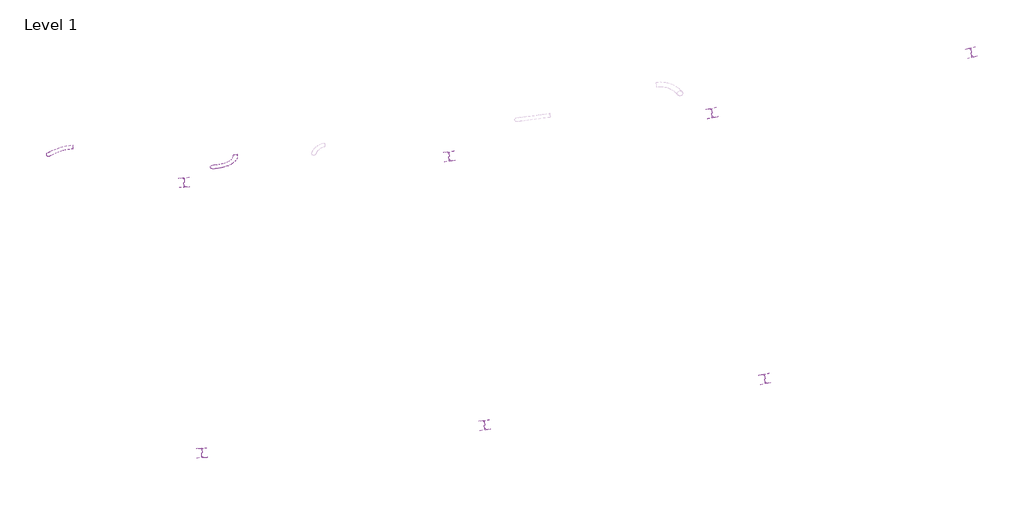
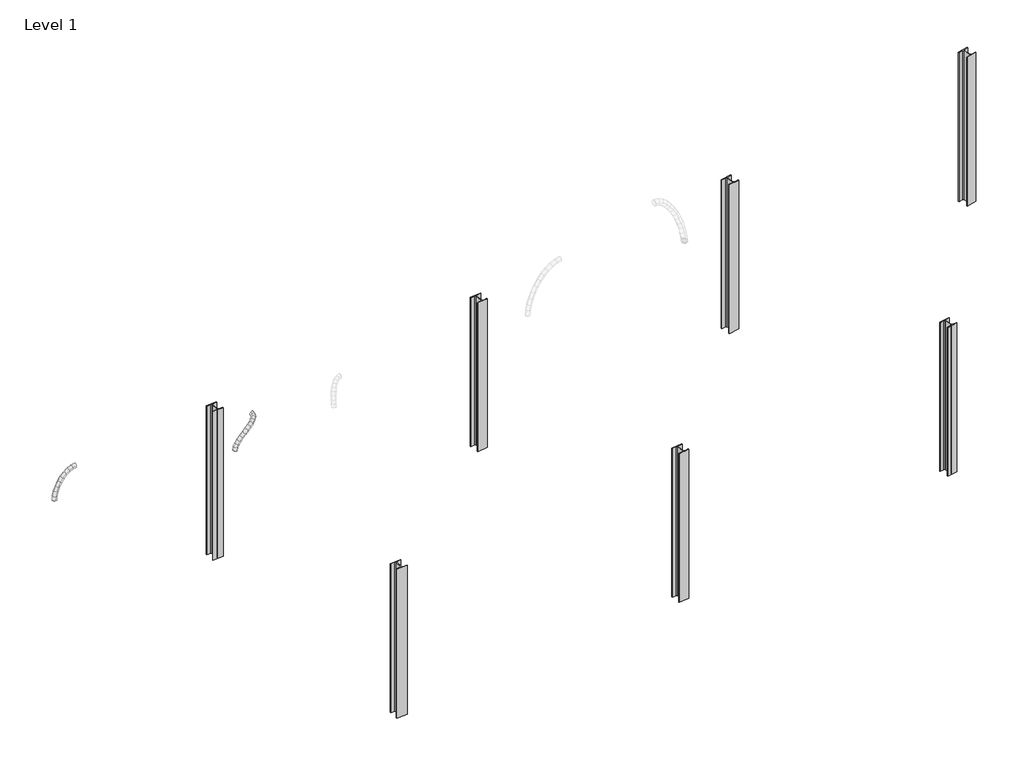
# One storey, part 1 of 3: 7 columns, 2 duct segments.
"""IFC4 building model written with IfcOpenShell, lengths in millimetres."""

import ifcopenshell
import ifcopenshell.guid

model = None  # the IFC model being written
_history = None  # IfcOwnerHistory: only IFC2X3 demands one
_inside = {}  # id of a spatial element -> (the spatial element, [elements in it])
_under = {}  # id of a project, library or spatial element -> (it, [spatial elements below it])
_declared = {}  # id of a project -> (the project, [libraries it declares])
_typed = {}  # id of a type object -> (the type object, [elements of that type])
_made_of = {}  # id of a material, layer set ... -> (it, [elements and type objects made of it])


def new_model(schema):
    """Start an empty IFC model of exactly this schema.

    Asked for "IFC4X3", IfcOpenShell would pick the latest addendum, in which some entities
    have other attributes; the version numbers below select the first issue.
    IFC2X3 requires an IfcOwnerHistory on every rooted entity: one is made here for all.
    """
    global model, _history
    if schema == "IFC4X3":
        model = ifcopenshell.file(schema_version=(4, 3, 0, 0))
    else:
        model = ifcopenshell.file(schema=schema)
    _inside.clear()
    _under.clear()
    _declared.clear()
    _typed.clear()
    _made_of.clear()
    _history = None
    if model.schema == "IFC2X3":
        org = make("IfcOrganization", Name="unknown")
        user = make(
            "IfcPersonAndOrganization",
            ThePerson=make("IfcPerson", FamilyName="unknown"),
            TheOrganization=org,
        )
        app = make(
            "IfcApplication",
            ApplicationDeveloper=org,
            Version="unknown",
            ApplicationFullName="unknown",
            ApplicationIdentifier="unknown",
        )
        _history = make(
            "IfcOwnerHistory",
            OwningUser=user,
            OwningApplication=app,
            ChangeAction="ADDED",
            CreationDate=0,
        )
    return model


def make(cls, **values):
    """One entity of the class cls with the attributes given. An attribute that is None is left unset."""
    return model.create_entity(
        cls, **{name: value for name, value in values.items() if value is not None}
    )


def rooted(cls, **values):
    """An entity with a GlobalId (a new one), such as an element, a storey or a relation."""
    return make(cls, GlobalId=ifcopenshell.guid.new(), OwnerHistory=_history, **values)


def si_unit(unit_type, name, prefix=None):
    """IfcSIUnit, for example si_unit("LENGTHUNIT", "METRE", prefix="MILLI")."""
    return make("IfcSIUnit", UnitType=unit_type, Prefix=prefix, Name=name)


def assignment(units):
    """IfcUnitAssignment: the units of a project."""
    return None if units is None else make("IfcUnitAssignment", Units=units)


def point(xyz):
    """IfcCartesianPoint."""
    return None if xyz is None else make("IfcCartesianPoint", Coordinates=xyz)


def direction(xyz):
    """IfcDirection."""
    return None if xyz is None else make("IfcDirection", DirectionRatios=xyz)


def frame(location, z_axis=None, x_axis=None):
    """IfcAxis2Placement3D, a coordinate frame: its origin and axes. An axis left out is left unset."""
    return make(
        "IfcAxis2Placement3D",
        Location=point(location),
        Axis=direction(z_axis),
        RefDirection=direction(x_axis),
    )


def frame_2d(location, x_axis=None):
    """IfcAxis2Placement2D, a coordinate frame in the plane: its origin and x axis."""
    return make(
        "IfcAxis2Placement2D", Location=point(location), RefDirection=direction(x_axis)
    )


def origin():
    """The frame at (0, 0, 0) with its axes left unset."""
    return frame((0.0, 0.0, 0.0))


def place(relative_to, where):
    """IfcLocalPlacement: puts the frame where relative to a parent placement (None: the world)."""
    return make(
        "IfcLocalPlacement", PlacementRelTo=relative_to, RelativePlacement=where
    )


def context(
    kind, dimensions, precision=None, world=None, true_north=None, identifier=None
):
    """IfcGeometricRepresentationContext, for example the 3D "Model" context."""
    return make(
        "IfcGeometricRepresentationContext",
        ContextIdentifier=identifier,
        ContextType=kind,
        CoordinateSpaceDimension=dimensions,
        Precision=precision,
        WorldCoordinateSystem=world,
        TrueNorth=true_north,
    )


def project(units=None, contexts=None):
    """IfcProject with its units and contexts."""
    return rooted(
        "IfcProject",
        Name="project",
        RepresentationContexts=contexts,
        UnitsInContext=assignment(units),
    )


def spatial(cls, under=None, at=None, **own):
    """A site, building, storey or space (cls), placed at a placement, below another one or the project."""
    s = rooted(cls, ObjectPlacement=at, **own)
    if under is not None:
        _under.setdefault(under.id(), (under, []))[1].append(s)
    return s


def polyline(points):
    """IfcPolyline through the points."""
    return make("IfcPolyline", Points=[point(p) for p in points])


def circle_curve(where, radius):
    """IfcCircle in the frame where."""
    return make("IfcCircle", Position=where, Radius=radius)


def ellipse_curve(where, semi_axis1, semi_axis2):
    """IfcEllipse in the frame where."""
    return make(
        "IfcEllipse", Position=where, SemiAxis1=semi_axis1, SemiAxis2=semi_axis2
    )


def trimmed(basis, trim1, trim2, sense, master):
    """IfcTrimmedCurve: the piece of a basis curve between two trims."""
    return make(
        "IfcTrimmedCurve",
        BasisCurve=basis,
        Trim1=trim1,
        Trim2=trim2,
        SenseAgreement=sense,
        MasterRepresentation=master,
    )


def segment(curve, same_sense, transition):
    """IfcCompositeCurveSegment."""
    return make(
        "IfcCompositeCurveSegment",
        Transition=transition,
        SameSense=same_sense,
        ParentCurve=curve,
    )


def composite_curve(segments, self_intersect=None):
    """IfcCompositeCurve: segments joined end to end."""
    return make("IfcCompositeCurve", Segments=segments, SelfIntersect=self_intersect)


def outline(outer, holes=None, kind="AREA"):
    """IfcArbitraryClosedProfileDef: a profile drawn as a closed curve; with holes, ...WithVoids."""
    if holes is None:
        return make("IfcArbitraryClosedProfileDef", ProfileType=kind, OuterCurve=outer)
    return make(
        "IfcArbitraryProfileDefWithVoids",
        ProfileType=kind,
        OuterCurve=outer,
        InnerCurves=holes,
    )


def extrude(swept, where, along, depth):
    """IfcExtrudedAreaSolid: the profile swept, set in the frame where, extruded along a direction by depth."""
    return make(
        "IfcExtrudedAreaSolid",
        SweptArea=swept,
        Position=where,
        ExtrudedDirection=direction(along),
        Depth=depth,
    )


def shape(context_of_items, identifier, shape_type, items):
    """IfcShapeRepresentation: the items that make up one representation, for example the "Body"."""
    return make(
        "IfcShapeRepresentation",
        ContextOfItems=context_of_items,
        RepresentationIdentifier=identifier,
        RepresentationType=shape_type,
        Items=items,
    )


def source(mapping_origin, context_of_items, identifier, shape_type, items):
    """IfcRepresentationMap: a shape defined once, which mapped items show again and again."""
    return make(
        "IfcRepresentationMap",
        MappingOrigin=mapping_origin,
        MappedRepresentation=shape(context_of_items, identifier, shape_type, items),
    )


def transform(
    local_origin,
    x_axis=None,
    y_axis=None,
    z_axis=None,
    scale=None,
    scale2=None,
    scale3=None,
    uniform=True,
):
    """IfcCartesianTransformationOperator3D, or its non-uniform kind. x_axis, y_axis, z_axis: its Axis1, 2, 3."""
    if uniform:
        return make(
            "IfcCartesianTransformationOperator3D",
            Axis1=direction(x_axis),
            Axis2=direction(y_axis),
            LocalOrigin=point(local_origin),
            Scale=scale,
            Axis3=direction(z_axis),
        )
    return make(
        "IfcCartesianTransformationOperator3DnonUniform",
        Axis1=direction(x_axis),
        Axis2=direction(y_axis),
        LocalOrigin=point(local_origin),
        Scale=scale,
        Axis3=direction(z_axis),
        Scale2=scale2,
        Scale3=scale3,
    )


def mapped(mapping_source, mapping_target):
    """IfcMappedItem: shows the shape of a source again, moved by a transform."""
    return make(
        "IfcMappedItem", MappingSource=mapping_source, MappingTarget=mapping_target
    )


def made_of(thing, what):
    """Note that an element or type object is made of a material, layer set ...; save() writes the relation."""
    if what is not None:
        _made_of.setdefault(what.id(), (what, []))[1].append(thing)
    return thing


def element(
    cls,
    number,
    at=None,
    inside=None,
    cuts=None,
    type_object=None,
    material=None,
    context=None,
    identifier="Body",
    shape_type=None,
    held_by="IfcProductDefinitionShape",
    body=None,
    shapes=None,
    **own,
):
    """One element of the class cls, such as IfcWall. Its Tag is "e" and its number.

    at: its placement. inside: the storey or other place that contains it. cuts: it is an
    opening in that element (IfcRelVoidsElement). A single representation is given by context,
    identifier, shape_type and body (its items); several are given by shapes. held_by: the class
    of the entity that holds the representations. save() writes the other relations.
    """
    e = rooted(cls, Tag="e%d" % number, ObjectPlacement=at, **own)
    if body is not None:
        shapes = [shape(context, identifier, shape_type, body)]
    if shapes is not None:
        e.Representation = make(held_by, Representations=shapes)
    if inside is not None:
        _inside.setdefault(inside.id(), (inside, []))[1].append(e)
    if cuts is not None:
        rooted(
            "IfcRelVoidsElement", RelatingBuildingElement=cuts, RelatedOpeningElement=e
        )
    if type_object is not None:
        _typed.setdefault(type_object.id(), (type_object, []))[1].append(e)
    return made_of(e, material)


def aggregate(whole, parts):
    """IfcRelAggregates: a whole, such as a stair, and the parts it consists of."""
    return rooted("IfcRelAggregates", RelatingObject=whole, RelatedObjects=parts)


def save(model, path):
    """Write the relations noted so far, then the file.

    IfcRelAggregates (storeys below a building ...), IfcRelContainedInSpatialStructure (elements
    in a storey), IfcRelDefinesByType, IfcRelAssociatesMaterial and IfcRelDeclares: one each for
    every whole, place, type object, material and project.
    """
    for whole, parts in _under.values():
        aggregate(whole, parts)
    for where, things in _inside.values():
        rooted(
            "IfcRelContainedInSpatialStructure",
            RelatedElements=things,
            RelatingStructure=where,
        )
    for kind, things in _typed.values():
        rooted("IfcRelDefinesByType", RelatedObjects=things, RelatingType=kind)
    for what, things in _made_of.values():
        rooted("IfcRelAssociatesMaterial", RelatedObjects=things, RelatingMaterial=what)
    for by, libraries in _declared.values():
        rooted("IfcRelDeclares", RelatingContext=by, RelatedDefinitions=libraries)
    model.write(path)


def plane_surface(at):
    """IfcPlane: the flat surface through the origin of the frame at, square to its z axis."""
    return make("IfcPlane", Position=at)


def cylinder_surface(at, radius):
    """IfcCylindricalSurface: all points at the distance radius from the z axis of the frame at."""
    return make("IfcCylindricalSurface", Position=at, Radius=radius)


def advanced_brep(points, edges, surfaces, faces):
    """IfcAdvancedBrep: a solid bounded by faces that lie on surfaces and meet in shared edges.

    An edge is (start, end): straight between two places in points (the first is 0);
    or (start, end, curve); or (start, end, curve, False) where it runs against its curve.
    A face is (place in surfaces, loops), or (place, loops, False) where it looks against
    its surface's normal. A loop lists edges by number (the first is 1), with a minus sign
    where the edge is run from its end to its start. The first loop is the outer one.
    """
    corners = [point(p) for p in points]
    vertices = [make("IfcVertexPoint", VertexGeometry=c) for c in corners]
    made = []
    for start, end, *more in edges:
        made.append(
            make(
                "IfcEdgeCurve",
                EdgeStart=vertices[start],
                EdgeEnd=vertices[end],
                EdgeGeometry=more[0] if more else make("IfcPolyline", Points=[corners[start], corners[end]]),
                SameSense=more[1] if len(more) > 1 else True,
            )
        )
    hull = []
    for where, loops, *sense in faces:
        bounds = []
        for j, loop in enumerate(loops):
            ring = [make("IfcOrientedEdge", EdgeElement=made[abs(k) - 1], Orientation=k > 0) for k in loop]
            bounds.append(
                make(
                    "IfcFaceOuterBound" if j == 0 else "IfcFaceBound",
                    Bound=make("IfcEdgeLoop", EdgeList=ring),
                    Orientation=True,
                )
            )
        hull.append(make("IfcAdvancedFace", Bounds=bounds, FaceSurface=surfaces[where], SameSense=sense[0] if sense else True))
    return make("IfcAdvancedBrep", Outer=make("IfcClosedShell", CfsFaces=hull))


def w_wide_flange_column1_w14x120_241bbdc2(model_context):
    return source(origin(), model_context, "Body", "SweptSolid", [
        extrude(outline(composite_curve([segment(polyline([(186.69, 184.15), (186.69, 160.274), (40.767, 160.274)]), True, "CONTINUOUS"), segment(trimmed(circle_curve(frame_2d((40.767, 127.0)), 33.274), [point((40.767, 160.274))], [point((7.493, 127.0))], True, "CARTESIAN"), True, "CONTINUOUS"), segment(polyline([(7.493, 127.0), (7.493, -127.0)]), True, "CONTINUOUS"), segment(trimmed(circle_curve(frame_2d((40.767, -127.0)), 33.274), [point((7.493, -127.0))], [point((40.767, -160.274))], True, "CARTESIAN"), True, "CONTINUOUS"), segment(polyline([(40.767, -160.274), (186.69, -160.274), (186.69, -184.15), (-186.69, -184.15), (-186.69, -160.274), (-40.767, -160.274)]), True, "CONTINUOUS"), segment(trimmed(circle_curve(frame_2d((-40.767, -127.0)), 33.274), [point((-40.767, -160.274))], [point((-7.493, -127.0))], True, "CARTESIAN"), True, "CONTINUOUS"), segment(polyline([(-7.493, -127.0), (-7.493, 127.0)]), True, "CONTINUOUS"), segment(trimmed(circle_curve(frame_2d((-40.767, 127.0)), 33.274), [point((-7.493, 127.0))], [point((-40.767, 160.274))], True, "CARTESIAN"), True, "CONTINUOUS"), segment(polyline([(-40.767, 160.274), (-186.69, 160.274), (-186.69, 184.15), (186.69, 184.15)]), True, "CONTINUOUS")], self_intersect=False)), frame((0.0, 0.0, 9144.0), z_axis=(0.0, 0.0, 1.0), x_axis=(1.0, 0.0, 0.0)), (0.0, 0.0, 1.0), 5486.4),
    ])


model = new_model("IFC4")

# Units and contexts
model_context = context("Model", 3, world=origin())
ifc_project = project(units=[si_unit("LENGTHUNIT", "METRE", prefix="MILLI")], contexts=[model_context])

# Site, building, storey
site = spatial("IfcSite", under=ifc_project)
building = spatial("IfcBuilding", under=site)
storey = spatial("IfcBuildingStorey", under=building, Name="Level 1", Elevation=0.0)

# Columns
placement = place(None, origin())
w_wide_flange_column1_w14x120_shape = w_wide_flange_column1_w14x120_241bbdc2(model_context)
element("IfcColumn", 1, ObjectType="W-Wide Flange-Column1 : W14X120", at=placement, inside=storey, context=model_context, shape_type="MappedRepresentation", body=[
    mapped(w_wide_flange_column1_w14x120_shape, transform((50697.9525321, 58874.0057575, 0.0), x_axis=(0.9978589232386037, 0.065403129230139, 0.0), y_axis=(-0.065403129230139, 0.9978589232386037, 0.0), z_axis=(0.0, 0.0, 1.0))),
])
element("IfcColumn", 2, ObjectType="W-Wide Flange-Column1 : W14X120", at=placement, inside=storey, context=model_context, shape_type="MappedRepresentation", body=[
    mapped(w_wide_flange_column1_w14x120_shape, transform((59812.3806883, 69814.7042697, 0.0), x_axis=(0.9914448613738108, 0.13052619222004747, 0.0), y_axis=(-0.13052619222004747, 0.9914448613738108, 0.0), z_axis=(0.0, 0.0, 1.0))),
])
element("IfcColumn", 3, ObjectType="W-Wide Flange-Column1 : W14X120", at=placement, inside=storey, context=model_context, shape_type="MappedRepresentation", body=[
    mapped(w_wide_flange_column1_w14x120_shape, transform((61117.6426105, 59900.2556559, 0.0), x_axis=(0.9914448613738108, 0.13052619222004747, 0.0), y_axis=(-0.13052619222004747, 0.9914448613738108, 0.0), z_axis=(0.0, 0.0, 1.0))),
])
element("IfcColumn", 4, ObjectType="W-Wide Flange-Column1 : W14X120", at=placement, inside=storey, context=model_context, shape_type="MappedRepresentation", body=[
    mapped(w_wide_flange_column1_w14x120_shape, transform((69497.0001577, 71413.6414152, 0.0), x_axis=(0.9807852804032312, 0.1950903220161241, 0.0), y_axis=(-0.1950903220161241, 0.9807852804032312, 0.0), z_axis=(0.0, 0.0, 1.0))),
])
element("IfcColumn", 5, ObjectType="W-Wide Flange-Column1 : W14X120", at=placement, inside=storey, context=model_context, shape_type="MappedRepresentation", body=[
    mapped(w_wide_flange_column1_w14x120_shape, transform((79056.3086207, 73642.5595324, 0.0), x_axis=(0.9659258262890681, 0.25881904510252196, 0.0), y_axis=(-0.25881904510252196, 0.9659258262890681, 0.0), z_axis=(0.0, 0.0, 1.0))),
])
element("IfcColumn", 6, ObjectType="W-Wide Flange-Column1 : W14X120", at=placement, inside=storey, context=model_context, shape_type="MappedRepresentation", body=[
    mapped(w_wide_flange_column1_w14x120_shape, transform((71447.9033779, 61605.7886112, 0.0), x_axis=(0.9807852804032312, 0.1950903220161241, 0.0), y_axis=(-0.1950903220161241, 0.9807852804032312, 0.0), z_axis=(0.0, 0.0, 1.0))),
])
element("IfcColumn", 7, ObjectType="W-Wide Flange-Column1 : W14X120", at=placement, inside=storey, context=model_context, shape_type="MappedRepresentation", body=[
    mapped(w_wide_flange_column1_w14x120_shape, transform((50043.9212398, 68852.5949899, 0.0), x_axis=(0.9978589232386037, 0.065403129230139, 0.0), y_axis=(-0.065403129230139, 0.9978589232386037, 0.0), z_axis=(0.0, 0.0, 1.0))),
])

# Duct segments
element("IfcDuctSegment", 8, ObjectType="Flex - Round", at=placement, inside=storey, context=model_context, shape_type="AdvancedBrep", body=[
    advanced_brep(
    [(51168.4264894, 69423.9819895, 12307.575), (51092.2264894, 69347.7819895, 12307.575), (51016.0264894, 69423.9819895, 12307.575), (51092.2264894, 69500.1819895, 12307.575), (51168.4264894, 69423.9819895, 12313.0663084), (51092.2264894, 69347.7819895, 12320.918666), (51016.0264894, 69423.9819895, 12327.8139791), (51092.2264894, 69500.1819895, 12319.9616215), (51976.8059535, 69887.0305194, 13041.5296548), (51871.4527395, 69873.1605056, 13059.4517924), (51889.2215508, 69875.499814, 13165.7140952), (51994.5747648, 69889.3698278, 13147.7919576), (51182.7000824, 69424.9082689, 12386.1232557), (51110.0863536, 69348.9409987, 12412.3313295), (51036.9081605, 69425.3370977, 12434.6932453), (51109.5218894, 69501.304368, 12408.4851715), (51223.6041441, 69428.4210516, 12470.7063417), (51159.5410001, 69353.1880934, 12514.5956634), (51092.9325593, 69430.1483934, 12550.5427805), (51156.9957033, 69505.3813516, 12506.6534588), (51288.9391245, 69435.8488802, 12557.0404322), (51234.1628389, 69361.67173, 12613.2014721), (51173.4932375, 69439.3072071, 12656.9962123), (51228.2695231, 69513.4843573, 12600.8351723), (51373.8859851, 69448.4791835, 12642.3019392), (51327.4936669, 69375.5486013, 12706.8780011), (51270.6032355, 69453.7459834, 12754.4659095), (51316.9955536, 69526.6765655, 12689.8898475), (51472.0204763, 69467.4797481, 12723.6444774), (51433.2382632, 69396.0226162, 12794.5284668), (51377.8808044, 69474.5168088, 12843.3870384), (51416.6630176, 69545.9739406, 12772.503049), (51576.7014197, 69493.9908677, 12798.9627951), (51545.2529794, 69424.3910608, 12875.1234607), (51489.161125, 69502.6992629, 12923.4536319), (51520.6095652, 69572.2990698, 12847.2929663), (51681.3579509, 69529.1706089, 12866.5914087), (51657.5862927, 69462.1513119, 12947.7127788), (51598.209063, 69539.3551524, 12993.9199543), (51621.9807212, 69606.3744495, 12912.7985842), (51779.561073, 69574.2562394, 12925.1221023), (51764.5401765, 69511.2544684, 13011.4590719), (51698.6476172, 69585.4670829, 13053.7830026), (51713.6685138, 69648.4688539, 12967.446033), (51865.0317331, 69630.7015392, 12973.3102482), (51860.5694324, 69574.6727238, 13065.6001278), (51783.9498426, 69641.8011475, 13101.8761854), (51788.4121433, 69697.829963, 13009.5863057), (51931.4504104, 69700.4299393, 13009.9445374), (51939.1327839, 69657.1509817, 13108.9330073), (51847.6292615, 69708.6537886, 13136.9995926), (51839.946888, 69751.9327462, 13038.0111227), (51971.5041654, 69785.4348086, 13033.3768829), (51988.58078, 69762.0929641, 13137.8611947), (51884.1928155, 69786.2515104, 13158.3900923), (51867.1162009, 69809.5933549, 13053.9057804), (51978.8794074, 69871.2810735, 13041.5296548), (51997.564446, 69866.6609448, 13147.7919576), (51890.8183283, 69863.3710844, 13165.7140952), (51872.1332898, 69867.991213, 13059.4517924)],
    [
        (0, 1, circle_curve(frame((51092.2264894, 69423.9819895, 12307.575), z_axis=(0.0, 0.0, -1.0), x_axis=(1.0, 0.0, 0.0)), 76.2)),
        (1, 2, circle_curve(frame((51092.2264894, 69423.9819895, 12307.575), z_axis=(0.0, 0.0, -1.0), x_axis=(1.0, 0.0, 0.0)), 76.2)),
        (2, 3, circle_curve(frame((51092.2264894, 69423.9819895, 12307.575), z_axis=(0.0, 0.0, -1.0), x_axis=(1.0, 0.0, 0.0)), 76.2)),
        (3, 0, circle_curve(frame((51092.2264894, 69423.9819895, 12307.575), z_axis=(0.0, 0.0, -1.0), x_axis=(1.0, 0.0, 0.0)), 76.2)),
        (0, 4),
        (4, 5, ellipse_curve(frame((51092.2264894, 69423.9819895, 12320.4401437), z_axis=(-0.09631767754478486, -0.006250499365662764, -0.9953310184305815), x_axis=(0.9932417901406138, 0.06445605144846851, -0.09652027636689438)), 76.5574453, 76.2)),
        (5, 1),
        (5, 6, ellipse_curve(frame((51092.2264894, 69423.9819895, 12320.4401437), z_axis=(-0.09631767754478486, -0.006250499365662764, -0.9953310184305815), x_axis=(0.9932417901406138, 0.06445605144846851, -0.09652027636689438)), 76.5574453, 76.2)),
        (6, 2),
        (6, 7, ellipse_curve(frame((51092.2264894, 69423.9819895, 12320.4401437), z_axis=(-0.09631767754478486, -0.006250499365662764, -0.9953310184305815), x_axis=(0.9932417901406138, 0.06445605144846851, -0.09652027636689438)), 76.5574453, 76.2)),
        (7, 3),
        (7, 4, ellipse_curve(frame((51092.2264894, 69423.9819895, 12320.4401437), z_axis=(-0.09631767754478486, -0.006250499365662764, -0.9953310184305815), x_axis=(0.9932417901406138, 0.06445605144846851, -0.09652027636689438)), 76.5574453, 76.2)),
        (8, 9, circle_curve(frame((51933.0137522, 69881.2651667, 13103.621875), z_axis=(-0.13052619222039535, 0.9914448613737652, 0.0), x_axis=(0.5747008054323026, 0.07566079640085344, -0.8148585325830805)), 76.2)),
        (9, 10, circle_curve(frame((51933.0137522, 69881.2651667, 13103.621875), z_axis=(-0.13052619222039535, 0.9914448613737652, 0.0), x_axis=(0.5747008054323026, 0.07566079640085344, -0.8148585325830805)), 76.2)),
        (10, 11, circle_curve(frame((51933.0137522, 69881.2651667, 13103.621875), z_axis=(-0.13052619222039535, 0.9914448613737652, 0.0), x_axis=(0.5747008054323026, 0.07566079640085344, -0.8148585325830805)), 76.2)),
        (11, 8, circle_curve(frame((51933.0137522, 69881.2651667, 13103.621875), z_axis=(-0.13052619222039535, 0.9914448613737652, 0.0), x_axis=(0.5747008054323026, 0.07566079640085344, -0.8148585325830805)), 76.2)),
        (4, 12),
        (12, 13, ellipse_curve(frame((51109.8041215, 69425.1226833, 12410.4082505), z_axis=(-0.3160345798820525, -0.02511197558409445, -0.9484152745506781), x_axis=(0.9435048554020643, 0.09662798879562944, -0.3169568103291704)), 76.8414929, 76.2)),
        (13, 5),
        (13, 14, ellipse_curve(frame((51109.8041215, 69425.1226833, 12410.4082505), z_axis=(-0.3160345798820525, -0.02511197558409445, -0.9484152745506781), x_axis=(0.9435048554020643, 0.09662798879562944, -0.3169568103291704)), 76.8414929, 76.2)),
        (14, 6),
        (14, 15, ellipse_curve(frame((51109.8041215, 69425.1226833, 12410.4082505), z_axis=(-0.3160345798820525, -0.02511197558409445, -0.9484152745506781), x_axis=(0.9435048554020643, 0.09662798879562944, -0.3169568103291704)), 76.8414929, 76.2)),
        (15, 7),
        (15, 12, ellipse_curve(frame((51109.8041215, 69425.1226833, 12410.4082505), z_axis=(-0.3160345798820525, -0.02511197558409445, -0.9484152745506781), x_axis=(0.9435048554020643, 0.09662798879562944, -0.3169568103291704)), 76.8414929, 76.2)),
        (12, 16),
        (16, 17, ellipse_curve(frame((51158.2683517, 69429.2847225, 12510.6245611), z_axis=(-0.5211367058988172, -0.053167539436947325, -0.8518155589769125), x_axis=(0.8382093189180972, 0.156029624271139, -0.522551331477269)), 76.5808213, 76.2)),
        (17, 13),
        (17, 18, ellipse_curve(frame((51158.2683517, 69429.2847225, 12510.6245611), z_axis=(-0.5211367058988172, -0.053167539436947325, -0.8518155589769125), x_axis=(0.8382093189180972, 0.156029624271139, -0.522551331477269)), 76.5808213, 76.2)),
        (18, 14),
        (18, 19, ellipse_curve(frame((51158.2683517, 69429.2847225, 12510.6245611), z_axis=(-0.5211367058988172, -0.053167539436947325, -0.8518155589769125), x_axis=(0.8382093189180972, 0.156029624271139, -0.522551331477269)), 76.5808213, 76.2)),
        (19, 15),
        (19, 16, ellipse_curve(frame((51158.2683517, 69429.2847225, 12510.6245611), z_axis=(-0.5211367058988172, -0.053167539436947325, -0.8518155589769125), x_axis=(0.8382093189180972, 0.156029624271139, -0.522551331477269)), 76.5808213, 76.2)),
        (16, 20),
        (20, 21, ellipse_curve(frame((51231.216181, 69437.5780436, 12607.0183222), z_axis=(-0.6535881241784717, -0.08661825149066223, -0.7518775448446158), x_axis=(0.714530641317517, 0.256919878154599, -0.6507212451022358)), 76.3869118, 76.2)),
        (21, 17),
        (21, 22, ellipse_curve(frame((51231.216181, 69437.5780436, 12607.0183222), z_axis=(-0.6535881241784717, -0.08661825149066223, -0.7518775448446158), x_axis=(0.714530641317517, 0.256919878154599, -0.6507212451022358)), 76.3869118, 76.2)),
        (22, 18),
        (22, 23, ellipse_curve(frame((51231.216181, 69437.5780436, 12607.0183222), z_axis=(-0.6535881241784717, -0.08661825149066223, -0.7518775448446158), x_axis=(0.714530641317517, 0.256919878154599, -0.6507212451022358)), 76.3869118, 76.2)),
        (23, 19),
        (23, 20, ellipse_curve(frame((51231.216181, 69437.5780436, 12607.0183222), z_axis=(-0.6535881241784717, -0.08661825149066223, -0.7518775448446158), x_axis=(0.714530641317517, 0.256919878154599, -0.6507212451022358)), 76.3869118, 76.2)),
        (20, 24),
        (24, 25, ellipse_curve(frame((51322.2446103, 69451.1125834, 12698.3839243), z_axis=(-0.7327038984960289, -0.12607290707821578, -0.6687679860979954), x_axis=(0.5734535630944716, 0.41478859054690154, -0.706471114856347)), 76.3029014, 76.2)),
        (25, 21),
        (25, 26, ellipse_curve(frame((51322.2446103, 69451.1125834, 12698.3839243), z_axis=(-0.7327038984960289, -0.12607290707821578, -0.6687679860979954), x_axis=(0.5734535630944716, 0.41478859054690154, -0.706471114856347)), 76.3029014, 76.2)),
        (26, 22),
        (26, 27, ellipse_curve(frame((51322.2446103, 69451.1125834, 12698.3839243), z_axis=(-0.7327038984960289, -0.12607290707821578, -0.6687679860979954), x_axis=(0.5734535630944716, 0.41478859054690154, -0.706471114856347)), 76.3029014, 76.2)),
        (27, 23),
        (27, 24, ellipse_curve(frame((51322.2446103, 69451.1125834, 12698.3839243), z_axis=(-0.7327038984960289, -0.12607290707821578, -0.6687679860979954), x_axis=(0.5734535630944716, 0.41478859054690154, -0.706471114856347)), 76.3029014, 76.2)),
        (24, 28),
        (28, 29, ellipse_curve(frame((51424.9506404, 69470.9982784, 12783.5157579), z_axis=(-0.7790268546089955, -0.17456502386147457, -0.602199478779464), x_axis=(0.38727829655513335, 0.6213647488513383, -0.6811177357126058)), 76.2718435, 76.2)),
        (29, 25),
        (29, 30, ellipse_curve(frame((51424.9506404, 69470.9982784, 12783.5157579), z_axis=(-0.7790268546089955, -0.17456502386147457, -0.602199478779464), x_axis=(0.38727829655513335, 0.6213647488513383, -0.6811177357126058)), 76.2718435, 76.2)),
        (30, 26),
        (30, 31, ellipse_curve(frame((51424.9506404, 69470.9982784, 12783.5157579), z_axis=(-0.7790268546089955, -0.17456502386147457, -0.602199478779464), x_axis=(0.38727829655513335, 0.6213647488513383, -0.6811177357126058)), 76.2718435, 76.2)),
        (31, 27),
        (31, 28, ellipse_curve(frame((51424.9506404, 69470.9982784, 12783.5157579), z_axis=(-0.7790268546089955, -0.17456502386147457, -0.602199478779464), x_axis=(0.38727829655513335, 0.6213647488513383, -0.6811177357126058)), 76.2718435, 76.2)),
        (28, 32),
        (32, 33, ellipse_curve(frame((51532.9312723, 69498.3450653, 12861.2082135), z_axis=(-0.8024634827890296, -0.2367603424025453, -0.547719726735792), x_axis=(0.15149357401677827, 0.806999043256463, -0.570790890970394)), 76.2724741, 76.2)),
        (33, 29),
        (33, 34, ellipse_curve(frame((51532.9312723, 69498.3450653, 12861.2082135), z_axis=(-0.8024634827890296, -0.2367603424025453, -0.547719726735792), x_axis=(0.15149357401677827, 0.806999043256463, -0.570790890970394)), 76.2724741, 76.2)),
        (34, 30),
        (34, 35, ellipse_curve(frame((51532.9312723, 69498.3450653, 12861.2082135), z_axis=(-0.8024634827890296, -0.2367603424025453, -0.547719726735792), x_axis=(0.15149357401677827, 0.806999043256463, -0.570790890970394)), 76.2724741, 76.2)),
        (35, 31),
        (35, 32, ellipse_curve(frame((51532.9312723, 69498.3450653, 12861.2082135), z_axis=(-0.8024634827890296, -0.2367603424025453, -0.547719726735792), x_axis=(0.15149357401677827, 0.806999043256463, -0.570790890970394)), 76.2724741, 76.2)),
        (32, 36),
        (36, 37, ellipse_curve(frame((51639.7835069, 69534.2628807, 12930.2556815), z_axis=(-0.8048364685833226, -0.3197400842879867, -0.5000045373172504), x_axis=(-0.08671065833968468, 0.8967814936867315, -0.43389424323363956)), 76.30749, 76.2)),
        (37, 33),
        (37, 38, ellipse_curve(frame((51639.7835069, 69534.2628807, 12930.2556815), z_axis=(-0.8048364685833226, -0.3197400842879867, -0.5000045373172504), x_axis=(-0.08671065833968468, 0.8967814936867315, -0.43389424323363956)), 76.30749, 76.2)),
        (38, 34),
        (38, 39, ellipse_curve(frame((51639.7835069, 69534.2628807, 12930.2556815), z_axis=(-0.8048364685833226, -0.3197400842879867, -0.5000045373172504), x_axis=(-0.08671065833968468, 0.8967814936867315, -0.43389424323363956)), 76.30749, 76.2)),
        (39, 35),
        (39, 36, ellipse_curve(frame((51639.7835069, 69534.2628807, 12930.2556815), z_axis=(-0.8048364685833226, -0.3197400842879867, -0.5000045373172504), x_axis=(-0.08671065833968468, 0.8967814936867315, -0.43389424323363956)), 76.30749, 76.2)),
        (36, 40),
        (40, 41, ellipse_curve(frame((51739.1043451, 69579.8616612, 12989.4525524), z_axis=(-0.7792162096624118, -0.43394853799753286, -0.4522286644709157), x_axis=(-0.2978259184454246, 0.8912390892158565, -0.3420418222320627)), 76.4090944, 76.2)),
        (41, 37),
        (41, 42, ellipse_curve(frame((51739.1043451, 69579.8616612, 12989.4525524), z_axis=(-0.7792162096624118, -0.43394853799753286, -0.4522286644709157), x_axis=(-0.2978259184454246, 0.8912390892158565, -0.3420418222320627)), 76.4090944, 76.2)),
        (42, 38),
        (42, 43, ellipse_curve(frame((51739.1043451, 69579.8616612, 12989.4525524), z_axis=(-0.7792162096624118, -0.43394853799753286, -0.4522286644709157), x_axis=(-0.2978259184454246, 0.8912390892158565, -0.3420418222320627)), 76.4090944, 76.2)),
        (43, 39),
        (43, 40, ellipse_curve(frame((51739.1043451, 69579.8616612, 12989.4525524), z_axis=(-0.7792162096624118, -0.43394853799753286, -0.4522286644709157), x_axis=(-0.2978259184454246, 0.8912390892158565, -0.3420418222320627)), 76.4090944, 76.2)),
        (40, 44),
        (44, 45, ellipse_curve(frame((51824.4907878, 69636.2513434, 13037.5932168), z_axis=(-0.7041660147765738, -0.5913286224194043, -0.39304030829069886), x_axis=(-0.49966744840142846, 0.8059750101377364, -0.3173904914163015)), 76.6694898, 76.2)),
        (45, 41),
        (45, 46, ellipse_curve(frame((51824.4907878, 69636.2513434, 13037.5932168), z_axis=(-0.7041660147765738, -0.5913286224194043, -0.39304030829069886), x_axis=(-0.49966744840142846, 0.8059750101377364, -0.3173904914163015)), 76.6694898, 76.2)),
        (46, 42),
        (46, 47, ellipse_curve(frame((51824.4907878, 69636.2513434, 13037.5932168), z_axis=(-0.7041660147765738, -0.5913286224194043, -0.39304030829069886), x_axis=(-0.49966744840142846, 0.8059750101377364, -0.3173904914163015)), 76.6694898, 76.2)),
        (47, 43),
        (47, 44, ellipse_curve(frame((51824.4907878, 69636.2513434, 13037.5932168), z_axis=(-0.7041660147765738, -0.5913286224194043, -0.39304030829069886), x_axis=(-0.49966744840142846, 0.8059750101377364, -0.3173904914163015)), 76.6694898, 76.2)),
        (44, 48),
        (48, 49, ellipse_curve(frame((51889.539836, 69704.5418639, 13073.472065), z_axis=(-0.5363116727490912, -0.7878245109880386, -0.30282392501176264), x_axis=(-0.7074245111556082, 0.6152774233262261, -0.34782790768034827)), 77.2369443, 76.2)),
        (49, 45),
        (49, 50, ellipse_curve(frame((51889.539836, 69704.5418639, 13073.472065), z_axis=(-0.5363116727490912, -0.7878245109880386, -0.30282392501176264), x_axis=(-0.7074245111556082, 0.6152774233262261, -0.34782790768034827)), 77.2369443, 76.2)),
        (50, 46),
        (50, 51, ellipse_curve(frame((51889.539836, 69704.5418639, 13073.472065), z_axis=(-0.5363116727490912, -0.7878245109880386, -0.30282392501176264), x_axis=(-0.7074245111556082, 0.6152774233262261, -0.34782790768034827)), 77.2369443, 76.2)),
        (51, 47),
        (51, 48, ellipse_curve(frame((51889.539836, 69704.5418639, 13073.472065), z_axis=(-0.5363116727490912, -0.7878245109880386, -0.30282392501176264), x_axis=(-0.7074245111556082, 0.6152774233262261, -0.34782790768034827)), 77.2369443, 76.2)),
        (48, 52),
        (52, 53, ellipse_curve(frame((51927.8484904, 69785.8431595, 13095.8834876), z_axis=(-0.2539694232227695, -0.9519478044338266, -0.17115755811973504), x_axis=(-0.869281899029314, 0.30224272620549875, -0.3911499897428829)), 77.5965914, 76.2)),
        (53, 49),
        (53, 54, ellipse_curve(frame((51927.8484904, 69785.8431595, 13095.8834876), z_axis=(-0.2539694232227695, -0.9519478044338266, -0.17115755811973504), x_axis=(-0.869281899029314, 0.30224272620549875, -0.3911499897428829)), 77.5965914, 76.2)),
        (54, 50),
        (54, 55, ellipse_curve(frame((51927.8484904, 69785.8431595, 13095.8834876), z_axis=(-0.2539694232227695, -0.9519478044338266, -0.17115755811973504), x_axis=(-0.869281899029314, 0.30224272620549875, -0.3911499897428829)), 77.5965914, 76.2)),
        (55, 51),
        (55, 52, ellipse_curve(frame((51927.8484904, 69785.8431595, 13095.8834876), z_axis=(-0.2539694232227695, -0.9519478044338266, -0.17115755811973504), x_axis=(-0.869281899029314, 0.30224272620549875, -0.3911499897428829)), 77.5965914, 76.2)),
        (52, 56),
        (56, 57, ellipse_curve(frame((51934.8488679, 69867.3260789, 13103.621875), z_axis=(0.02281354896807852, -0.9986140186542781, -0.04742977683517217), x_axis=(-0.9164473766326617, -0.0019310413576735263, -0.40015056783964104)), 76.7334121, 76.2)),
        (57, 53),
        (57, 58, ellipse_curve(frame((51934.8488679, 69867.3260789, 13103.621875), z_axis=(0.02281354896807852, -0.9986140186542781, -0.04742977683517217), x_axis=(-0.9164473766326617, -0.0019310413576735263, -0.40015056783964104)), 76.7334121, 76.2)),
        (58, 54),
        (58, 59, ellipse_curve(frame((51934.8488679, 69867.3260789, 13103.621875), z_axis=(0.02281354896807852, -0.9986140186542781, -0.04742977683517217), x_axis=(-0.9164473766326617, -0.0019310413576735263, -0.40015056783964104)), 76.7334121, 76.2)),
        (59, 55),
        (59, 56, ellipse_curve(frame((51934.8488679, 69867.3260789, 13103.621875), z_axis=(0.02281354896807852, -0.9986140186542781, -0.04742977683517217), x_axis=(-0.9164473766326617, -0.0019310413576735263, -0.40015056783964104)), 76.7334121, 76.2)),
        (56, 8),
        (11, 57),
        (10, 58),
        (9, 59),
    ],
    [
        plane_surface(frame((51092.2264894, 69347.7819895, 12307.575), z_axis=(0.0, 0.0, -1.0), x_axis=(1.0, 0.0, 0.0))),
        cylinder_surface(frame((51092.2264894, 69423.9819895, 12307.575), z_axis=(0.0, 0.0, -1.0), x_axis=(1.0, 0.0, 0.0)), 76.2),
        plane_surface(frame((51933.0137522, 69881.2651667, 13179.821875), z_axis=(-0.13052619222040104, 0.9914448613737645, 0.0), x_axis=(0.9914448613737645, 0.13052619222040104, 0.0))),
        cylinder_surface(frame((51092.2264894, 69423.9819895, 12320.4401437), z_axis=(-0.19173594416703815, -0.012442631798649646, -0.9813676725001175), x_axis=(0.9814458099847577, -0.0012040671647915765, -0.19173594416703812)), 76.2),
        cylinder_surface(frame((51109.8041215, 69425.1226833, 12410.4082505), z_axis=(-0.435056536762002, -0.03736203667547233, -0.899627638546145), x_axis=(0.9003543204050997, -0.0076475630226252875, -0.43509034982137446)), 76.2),
        cylinder_surface(frame((51158.2683517, 69429.2847225, 12510.6245611), z_axis=(-0.6020338555262282, -0.06844425888485121, -0.7955316588457862), x_axis=(0.7980193797868307, -0.01808800394630852, -0.6023602689403414)), 76.2),
        cylinder_surface(frame((51231.216181, 69437.5780436, 12607.0183222), z_axis=(-0.701943851312699, -0.10436835011284386, -0.7045438787605912), x_axis=(0.710297294027706, -0.02971357271734463, -0.7032743829354868)), 76.2),
        cylinder_surface(frame((51322.2446103, 69451.1125834, 12698.3839243), z_axis=(-0.7614877093330051, -0.14743742236813073, -0.6311883039317302), x_axis=(0.6423549405529348, -0.04140409331356675, -0.7652880708622846)), 76.2),
        cylinder_surface(frame((51424.9506404, 69470.9982784, 12783.5157579), z_axis=(-0.7950984064909467, -0.2013637657342114, -0.5720761818542135), x_axis=(0.5919862348435673, -0.0526907572610381, -0.8042238381539031)), 76.2),
        cylinder_surface(frame((51532.9312723, 69498.3450653, 12861.2082135), z_axis=(-0.8083035583714235, -0.27170697997788057, -0.5223223856541039), x_axis=(0.5565446436129712, -0.06314751131280223, -0.8284144201308368)), 76.2),
        cylinder_surface(frame((51639.7835069, 69534.2628807, 12930.2556815), z_axis=(-0.799101924138622, -0.3668723892788268, -0.47627803310964995), x_axis=(0.5347727448698782, -0.07179690657626409, -0.8419402090115516)), 76.2),
        cylinder_surface(frame((51739.1043451, 69579.8616612, 12989.4525524), z_axis=(-0.7550658265598512, -0.4986496761703849, -0.4257042377245723), x_axis=(0.527295491532616, -0.07596101804328277, -0.8462797340993136)), 76.2),
        cylinder_surface(frame((51824.4907878, 69636.2513434, 13037.5932168), z_axis=(-0.6446422042087945, -0.6767655018631916, -0.35556277088678645), x_axis=(0.536078423070622, -0.06858548628203899, -0.8413774155452305)), 76.2),
        cylinder_surface(frame((51889.539836, 69704.5418639, 13073.472065), z_axis=(-0.41358064009421036, -0.8777296493535199, -0.24195395591932478), x_axis=(0.5589439884113595, -0.034996709926131915, -0.8284665642698855)), 76.2),
        cylinder_surface(frame((51927.8484904, 69785.8431595, 13095.8834876), z_axis=(-0.08521627092010084, -0.9918994511620645, -0.09420013776458847), x_axis=(0.5757865664993499, 0.02813394189963552, -0.8171158492845906)), 76.2),
        cylinder_surface(frame((51934.8488679, 69867.3260789, 13103.621875), z_axis=(0.13052619222039535, -0.9914448613737652, 0.0), x_axis=(0.5747008054323026, 0.07566079640085344, -0.8148585325830805)), 76.2),
    ],
    [
        (0, [[1, 2, 3, 4]]),
        (1, [[-1, 5, 6, 7]]),
        (1, [[-2, -7, 8, 9]]),
        (1, [[-3, -9, 10, 11]]),
        (1, [[-4, -11, 12, -5]]),
        (2, [[13, 14, 15, 16]]),
        (3, [[-6, 17, 18, 19]]),
        (3, [[-8, -19, 20, 21]]),
        (3, [[-10, -21, 22, 23]]),
        (3, [[-12, -23, 24, -17]]),
        (4, [[-18, 25, 26, 27]]),
        (4, [[-20, -27, 28, 29]]),
        (4, [[-22, -29, 30, 31]]),
        (4, [[-24, -31, 32, -25]]),
        (5, [[-26, 33, 34, 35]]),
        (5, [[-28, -35, 36, 37]]),
        (5, [[-30, -37, 38, 39]]),
        (5, [[-32, -39, 40, -33]]),
        (6, [[-34, 41, 42, 43]]),
        (6, [[-36, -43, 44, 45]]),
        (6, [[-38, -45, 46, 47]]),
        (6, [[-40, -47, 48, -41]]),
        (7, [[-42, 49, 50, 51]]),
        (7, [[-44, -51, 52, 53]]),
        (7, [[-46, -53, 54, 55]]),
        (7, [[-48, -55, 56, -49]]),
        (8, [[-50, 57, 58, 59]]),
        (8, [[-52, -59, 60, 61]]),
        (8, [[-54, -61, 62, 63]]),
        (8, [[-56, -63, 64, -57]]),
        (9, [[-58, 65, 66, 67]]),
        (9, [[-60, -67, 68, 69]]),
        (9, [[-62, -69, 70, 71]]),
        (9, [[-64, -71, 72, -65]]),
        (10, [[-66, 73, 74, 75]]),
        (10, [[-68, -75, 76, 77]]),
        (10, [[-70, -77, 78, 79]]),
        (10, [[-72, -79, 80, -73]]),
        (11, [[-74, 81, 82, 83]]),
        (11, [[-76, -83, 84, 85]]),
        (11, [[-78, -85, 86, 87]]),
        (11, [[-80, -87, 88, -81]]),
        (12, [[-82, 89, 90, 91]]),
        (12, [[-84, -91, 92, 93]]),
        (12, [[-86, -93, 94, 95]]),
        (12, [[-88, -95, 96, -89]]),
        (13, [[-90, 97, 98, 99]]),
        (13, [[-92, -99, 100, 101]]),
        (13, [[-94, -101, 102, 103]]),
        (13, [[-96, -103, 104, -97]]),
        (14, [[-98, 105, 106, 107]]),
        (14, [[-100, -107, 108, 109]]),
        (14, [[-102, -109, 110, 111]]),
        (14, [[-104, -111, 112, -105]]),
        (15, [[-106, 113, -16, 114]]),
        (15, [[-108, -114, -15, 115]]),
        (15, [[-110, -115, -14, 116]]),
        (15, [[-112, -116, -13, -113]]),
    ],
),
])
element("IfcDuctSegment", 9, ObjectType="Flex - Round", at=placement, inside=storey, context=model_context, shape_type="AdvancedBrep", body=[
    advanced_brep(
    [(45126.3556237, 69881.2651667, 12307.575), (45050.1556237, 69805.0651667, 12307.575), (44973.9556237, 69881.2651667, 12307.575), (45050.1556237, 69957.4651667, 12307.575), (45126.3556237, 69881.2651667, 12313.2784342), (45050.1556237, 69805.0651667, 12321.4022592), (44973.9556237, 69881.2651667, 12323.7833249), (45050.1556237, 69957.4651667, 12315.6594999), (45946.6686733, 70134.3153429, 13030.6071857), (45946.6686733, 70229.1825501, 13081.725607), (45946.6686733, 70178.0641288, 13176.5928143), (45946.6686733, 70083.1969216, 13125.474393), (45141.7533276, 69889.6827036, 12424.2804717), (45068.3628736, 69815.0186117, 12452.658312), (44993.0506015, 69891.7039102, 12461.439008), (45066.4410555, 69966.3680022, 12433.0611677), (45185.1326809, 69912.2127507, 12540.667355), (45119.4743717, 69841.5645228, 12589.7905539), (45046.9710146, 69919.7086948, 12606.1075736), (45112.6293237, 69990.3569226, 12556.9843747), (45253.9403085, 69945.5868417, 12652.6933123), (45197.4047693, 69879.3634744, 12716.6693272), (45129.0028204, 69959.4969719, 12739.6638652), (45185.5383596, 70025.7203393, 12675.6878503), (45344.4236674, 69985.8121425, 12756.6431821), (45296.8546553, 69923.5749364, 12830.9201998), (45233.6311443, 70006.0105612, 12859.8638753), (45281.2001563, 70068.2477674, 12785.5868576), (45451.9199847, 70028.4452697, 12848.5566077), (45412.9640411, 69969.6240135, 12930.1981254), (45356.2513414, 70054.6418315, 12964.7087913), (45395.207285, 70113.4630877, 12883.0672736), (45571.3423051, 70068.931494, 12924.8287172), (45540.9341822, 70013.0080963, 13011.9295185), (45492.6829494, 70100.8944973, 13051.844316), (45523.0910723, 70156.817895, 12964.7435147), (45697.2884551, 70102.7681046, 12982.2222599), (45675.869918, 70049.2598432, 13073.4196071), (45639.0607241, 70140.2202549, 13118.5485309), (45660.4792611, 70193.7285164, 13027.3511838), (45824.316522, 70125.7331612, 13018.0451919), (45812.7793098, 70074.0113175, 13112.0291517), (45791.5591604, 70167.7900299, 13161.554311), (45803.0963726, 70219.5118737, 13067.5703511), (45943.7491236, 70134.3153429, 13030.6071857), (45940.6093464, 70083.1969216, 13125.474393), (45934.5370655, 70178.0641288, 13176.5928143), (45937.6768427, 70229.1825501, 13081.725607)],
    [
        (0, 1, circle_curve(frame((45050.1556237, 69881.2651667, 12307.575), z_axis=(0.0, 0.0, -1.0), x_axis=(1.0, 0.0, 0.0)), 76.2)),
        (1, 2, circle_curve(frame((45050.1556237, 69881.2651667, 12307.575), z_axis=(0.0, 0.0, -1.0), x_axis=(1.0, 0.0, 0.0)), 76.2)),
        (2, 3, circle_curve(frame((45050.1556237, 69881.2651667, 12307.575), z_axis=(0.0, 0.0, -1.0), x_axis=(1.0, 0.0, 0.0)), 76.2)),
        (3, 0, circle_curve(frame((45050.1556237, 69881.2651667, 12307.575), z_axis=(0.0, 0.0, -1.0), x_axis=(1.0, 0.0, 0.0)), 76.2)),
        (0, 4),
        (4, 5, ellipse_curve(frame((45050.1556237, 69881.2651667, 12318.5308796), z_axis=(-0.06871801703430311, -0.03756640949875729, -0.9969285827040194), x_axis=(0.8747500723822876, 0.47820383716510206, -0.07831603276312736)), 76.4347631, 76.2)),
        (5, 1),
        (5, 6, ellipse_curve(frame((45050.1556237, 69881.2651667, 12318.5308796), z_axis=(-0.06871801703430311, -0.03756640949875729, -0.9969285827040194), x_axis=(0.8747500723822876, 0.47820383716510206, -0.07831603276312736)), 76.4347631, 76.2)),
        (6, 2),
        (6, 7, ellipse_curve(frame((45050.1556237, 69881.2651667, 12318.5308796), z_axis=(-0.06871801703430311, -0.03756640949875729, -0.9969285827040194), x_axis=(0.8747500723822876, 0.47820383716510206, -0.07831603276312736)), 76.4347631, 76.2)),
        (7, 3),
        (7, 4, ellipse_curve(frame((45050.1556237, 69881.2651667, 12318.5308796), z_axis=(-0.06871801703430311, -0.03756640949875729, -0.9969285827040194), x_axis=(0.8747500723822876, 0.47820383716510206, -0.07831603276312736)), 76.4347631, 76.2)),
        (8, 9, circle_curve(frame((45946.6686733, 70156.1897358, 13103.6), z_axis=(1.0, 0.0, 0.0), x_axis=(0.0, -0.2870655243811556, -0.9579109482158413)), 76.2)),
        (9, 10, circle_curve(frame((45946.6686733, 70156.1897358, 13103.6), z_axis=(1.0, 0.0, 0.0), x_axis=(0.0, -0.2870655243811556, -0.9579109482158413)), 76.2)),
        (10, 11, circle_curve(frame((45946.6686733, 70156.1897358, 13103.6), z_axis=(1.0, 0.0, 0.0), x_axis=(0.0, -0.2870655243811556, -0.9579109482158413)), 76.2)),
        (11, 8, circle_curve(frame((45946.6686733, 70156.1897358, 13103.6), z_axis=(1.0, 0.0, 0.0), x_axis=(0.0, -0.2870655243811556, -0.9579109482158413)), 76.2)),
        (4, 12),
        (12, 13, ellipse_curve(frame((45067.4019645, 69890.6933069, 12442.8597398), z_axis=(-0.24208048403591495, -0.12761400910702309, -0.9618272734376844), x_axis=(0.8598612548607711, 0.43102130134720873, -0.27360420350246556)), 76.7560458, 76.2)),
        (13, 5),
        (13, 14, ellipse_curve(frame((45067.4019645, 69890.6933069, 12442.8597398), z_axis=(-0.24208048403591495, -0.12761400910702309, -0.9618272734376844), x_axis=(0.8598612548607711, 0.43102130134720873, -0.27360420350246556)), 76.7560458, 76.2)),
        (14, 6),
        (14, 15, ellipse_curve(frame((45067.4019645, 69890.6933069, 12442.8597398), z_axis=(-0.24208048403591495, -0.12761400910702309, -0.9618272734376844), x_axis=(0.8598612548607711, 0.43102130134720873, -0.27360420350246556)), 76.7560458, 76.2)),
        (15, 7),
        (15, 12, ellipse_curve(frame((45067.4019645, 69890.6933069, 12442.8597398), z_axis=(-0.24208048403591495, -0.12761400910702309, -0.9618272734376844), x_axis=(0.8598612548607711, 0.43102130134720873, -0.27360420350246556)), 76.7560458, 76.2)),
        (12, 16),
        (16, 17, ellipse_curve(frame((45116.0518477, 69915.9607227, 12573.3874643), z_axis=(-0.42763544407329346, -0.21334812823957647, -0.8784136287358629), x_axis=(0.8123862993433231, 0.3354565549059712, -0.47696687558978124)), 76.5894505, 76.2)),
        (17, 13),
        (17, 18, ellipse_curve(frame((45116.0518477, 69915.9607227, 12573.3874643), z_axis=(-0.42763544407329346, -0.21334812823957647, -0.8784136287358629), x_axis=(0.8123862993433231, 0.3354565549059712, -0.47696687558978124)), 76.5894505, 76.2)),
        (18, 14),
        (18, 19, ellipse_curve(frame((45116.0518477, 69915.9607227, 12573.3874643), z_axis=(-0.42763544407329346, -0.21334812823957647, -0.8784136287358629), x_axis=(0.8123862993433231, 0.3354565549059712, -0.47696687558978124)), 76.5894505, 76.2)),
        (19, 15),
        (19, 16, ellipse_curve(frame((45116.0518477, 69915.9607227, 12573.3874643), z_axis=(-0.42763544407329346, -0.21334812823957647, -0.8784136287358629), x_axis=(0.8123862993433231, 0.3354565549059712, -0.47696687558978124)), 76.5894505, 76.2)),
        (16, 20),
        (20, 21, ellipse_curve(frame((45191.4715644, 69952.5419068, 12696.1785888), z_axis=(-0.5706766792227911, -0.2640005399955803, -0.7775807627978522), x_axis=(0.7531539425983521, 0.20907867188404253, -0.623734917823079)), 76.4552316, 76.2)),
        (21, 17),
        (21, 22, ellipse_curve(frame((45191.4715644, 69952.5419068, 12696.1785888), z_axis=(-0.5706766792227911, -0.2640005399955803, -0.7775807627978522), x_axis=(0.7531539425983521, 0.20907867188404253, -0.623734917823079)), 76.4552316, 76.2)),
        (22, 18),
        (22, 23, ellipse_curve(frame((45191.4715644, 69952.5419068, 12696.1785888), z_axis=(-0.5706766792227911, -0.2640005399955803, -0.7775807627978522), x_axis=(0.7531539425983521, 0.20907867188404253, -0.623734917823079)), 76.4552316, 76.2)),
        (23, 19),
        (23, 20, ellipse_curve(frame((45191.4715644, 69952.5419068, 12696.1785888), z_axis=(-0.5706766792227911, -0.2640005399955803, -0.7775807627978522), x_axis=(0.7531539425983521, 0.20907867188404253, -0.623734917823079)), 76.4552316, 76.2)),
        (20, 24),
        (24, 25, ellipse_curve(frame((45289.0274058, 69995.9113519, 12808.2535287), z_axis=(-0.6806813284839914, -0.28511004427654657, -0.6748223408467551), x_axis=(0.6900852035954025, 0.059624532191602346, -0.7212678607421965)), 76.3906311, 76.2)),
        (25, 21),
        (25, 26, ellipse_curve(frame((45289.0274058, 69995.9113519, 12808.2535287), z_axis=(-0.6806813284839914, -0.28511004427654657, -0.6748223408467551), x_axis=(0.6900852035954025, 0.059624532191602346, -0.7212678607421965)), 76.3906311, 76.2)),
        (26, 22),
        (26, 27, ellipse_curve(frame((45289.0274058, 69995.9113519, 12808.2535287), z_axis=(-0.6806813284839914, -0.28511004427654657, -0.6748223408467551), x_axis=(0.6900852035954025, 0.059624532191602346, -0.7212678607421965)), 76.3906311, 76.2)),
        (27, 23),
        (27, 24, ellipse_curve(frame((45289.0274058, 69995.9113519, 12808.2535287), z_axis=(-0.6806813284839914, -0.28511004427654657, -0.6748223408467551), x_axis=(0.6900852035954025, 0.059624532191602346, -0.7212678607421965)), 76.3906311, 76.2)),
        (24, 28),
        (28, 29, ellipse_curve(frame((45404.085663, 70041.5435506, 12906.6326995), z_axis=(-0.7707616099340316, -0.28230062668244676, -0.5711680110323036), x_axis=(0.6163898505215764, -0.10355956324943726, -0.7806016711701137)), 76.371817, 76.2)),
        (29, 25),
        (29, 30, ellipse_curve(frame((45404.085663, 70041.5435506, 12906.6326995), z_axis=(-0.7707616099340316, -0.28230062668244676, -0.5711680110323036), x_axis=(0.6163898505215764, -0.10355956324943726, -0.7806016711701137)), 76.371817, 76.2)),
        (30, 26),
        (30, 31, ellipse_curve(frame((45404.085663, 70041.5435506, 12906.6326995), z_axis=(-0.7707616099340316, -0.28230062668244676, -0.5711680110323036), x_axis=(0.6163898505215764, -0.10355956324943726, -0.7806016711701137)), 76.371817, 76.2)),
        (31, 27),
        (31, 28, ellipse_curve(frame((45404.085663, 70041.5435506, 12906.6326995), z_axis=(-0.7707616099340316, -0.28230062668244676, -0.5711680110323036), x_axis=(0.6163898505215764, -0.10355956324943726, -0.7806016711701137)), 76.371817, 76.2)),
        (28, 32),
        (32, 33, ellipse_curve(frame((45532.0126272, 70084.9129957, 12988.3365166), z_axis=(-0.8492671945607192, -0.2567422705978809, -0.46133354390420156), x_axis=(0.5207659217450847, -0.2635694264299794, -0.8119938498537804)), 76.390909, 76.2)),
        (33, 29),
        (33, 34, ellipse_curve(frame((45532.0126272, 70084.9129957, 12988.3365166), z_axis=(-0.8492671945607192, -0.2567422705978809, -0.46133354390420156), x_axis=(0.5207659217450847, -0.2635694264299794, -0.8119938498537804)), 76.390909, 76.2)),
        (34, 30),
        (34, 35, ellipse_curve(frame((45532.0126272, 70084.9129957, 12988.3365166), z_axis=(-0.8492671945607192, -0.2567422705978809, -0.46133354390420156), x_axis=(0.5207659217450847, -0.2635694264299794, -0.8119938498537804)), 76.390909, 76.2)),
        (35, 31),
        (35, 32, ellipse_curve(frame((45532.0126272, 70084.9129957, 12988.3365166), z_axis=(-0.8492671945607192, -0.2567422705978809, -0.46133354390420156), x_axis=(0.5207659217450847, -0.2635694264299794, -0.8119938498537804)), 76.390909, 76.2)),
        (32, 36),
        (36, 37, ellipse_curve(frame((45668.1745896, 70121.4941798, 13050.3853954), z_axis=(-0.9191639051242704, -0.2051408080504545, -0.33623647093839715), x_axis=(0.39240573190139333, -0.4032668322895574, -0.826676238648528)), 76.4568405, 76.2)),
        (37, 33),
        (37, 38, ellipse_curve(frame((45668.1745896, 70121.4941798, 13050.3853954), z_axis=(-0.9191639051242704, -0.2051408080504545, -0.33623647093839715), x_axis=(0.39240573190139333, -0.4032668322895574, -0.826676238648528)), 76.4568405, 76.2)),
        (38, 34),
        (38, 39, ellipse_curve(frame((45668.1745896, 70121.4941798, 13050.3853954), z_axis=(-0.9191639051242704, -0.2051408080504545, -0.33623647093839715), x_axis=(0.39240573190139333, -0.4032668322895574, -0.826676238648528)), 76.4568405, 76.2)),
        (39, 35),
        (39, 36, ellipse_curve(frame((45668.1745896, 70121.4941798, 13050.3853954), z_axis=(-0.9191639051242704, -0.2051408080504545, -0.33623647093839715), x_axis=(0.39240573190139333, -0.4032668322895574, -0.826676238648528)), 76.4568405, 76.2)),
        (36, 40),
        (40, 41, ellipse_curve(frame((45807.9378412, 70146.7615956, 13089.7997514), z_axis=(-0.9748056898678453, -0.12194223254948801, -0.18677247902761443), x_axis=(0.22297463942560755, -0.5101433081700157, -0.8306841248647844)), 76.5697204, 76.2)),
        (41, 37),
        (41, 42, ellipse_curve(frame((45807.9378412, 70146.7615956, 13089.7997514), z_axis=(-0.9748056898678453, -0.12194223254948801, -0.18677247902761443), x_axis=(0.22297463942560755, -0.5101433081700157, -0.8306841248647844)), 76.5697204, 76.2)),
        (42, 38),
        (42, 43, ellipse_curve(frame((45807.9378412, 70146.7615956, 13089.7997514), z_axis=(-0.9748056898678453, -0.12194223254948801, -0.18677247902761443), x_axis=(0.22297463942560755, -0.5101433081700157, -0.8306841248647844)), 76.5697204, 76.2)),
        (43, 39),
        (43, 40, ellipse_curve(frame((45807.9378412, 70146.7615956, 13089.7997514), z_axis=(-0.9748056898678453, -0.12194223254948801, -0.18677247902761443), x_axis=(0.22297463942560755, -0.5101433081700157, -0.8306841248647844)), 76.5697204, 76.2)),
        (40, 44),
        (44, 45, ellipse_curve(frame((45939.1430946, 70156.1897358, 13103.6), z_axis=(-0.9979940276422552, -0.03571261138933422, -0.052273608811174876), x_axis=(0.06330814158059515, -0.5629761352682932, -0.82404487155008)), 76.3531623, 76.2)),
        (45, 41),
        (45, 46, ellipse_curve(frame((45939.1430946, 70156.1897358, 13103.6), z_axis=(-0.9979940276422552, -0.03571261138933422, -0.052273608811174876), x_axis=(0.06330814158059515, -0.5629761352682932, -0.82404487155008)), 76.3531623, 76.2)),
        (46, 42),
        (46, 47, ellipse_curve(frame((45939.1430946, 70156.1897358, 13103.6), z_axis=(-0.9979940276422552, -0.03571261138933422, -0.052273608811174876), x_axis=(0.06330814158059515, -0.5629761352682932, -0.82404487155008)), 76.3531623, 76.2)),
        (47, 43),
        (47, 44, ellipse_curve(frame((45939.1430946, 70156.1897358, 13103.6), z_axis=(-0.9979940276422552, -0.03571261138933422, -0.052273608811174876), x_axis=(0.06330814158059515, -0.5629761352682932, -0.82404487155008)), 76.3531623, 76.2)),
        (44, 8),
        (11, 45),
        (10, 46),
        (9, 47),
    ],
    [
        plane_surface(frame((45050.1556237, 69805.0651667, 12307.575), z_axis=(0.0, 0.0, -1.0), x_axis=(1.0, 0.0, 0.0))),
        cylinder_surface(frame((45050.1556237, 69881.2651667, 12307.575), z_axis=(0.0, 0.0, -1.0), x_axis=(1.0, 0.0, 0.0)), 76.2),
        plane_surface(frame((45946.6686733, 70156.1897358, 13027.4), z_axis=(1.0, 0.0, 0.0), x_axis=(0.0, 1.0, 0.0))),
        cylinder_surface(frame((45050.1556237, 69881.2651667, 12318.5308796), z_axis=(-0.13701391065647692, -0.07490205475774983, -0.9877331980244899), x_axis=(0.9905556682697465, -0.005162978335706418, -0.1370139106564769)), 76.2),
        cylinder_surface(frame((45067.4019645, 69890.6933069, 12442.8597398), z_axis=(-0.3436396375499582, -0.17847700850056256, -0.9219857682964655), x_axis=(0.938580208283955, -0.03256211730547343, -0.3435213255887211)), 76.2),
        cylinder_surface(frame((45116.0518477, 69915.9607227, 12573.3874643), z_axis=(-0.5072822743131246, -0.2460495355220969, -0.8259081790593094), x_axis=(0.8593228681113003, -0.07210375355063259, -0.5063252482988365)), 76.2),
        cylinder_surface(frame((45191.4715644, 69952.5419068, 12696.1785888), z_axis=(-0.6302608880669694, -0.28018891099305093, -0.724061728811545), x_axis=(0.7706952754274137, -0.11310373336217841, -0.6270855905962123)), 76.2),
        cylinder_surface(frame((45289.0274058, 69995.9113519, 12808.2535287), z_axis=(-0.727704518550323, -0.2886082059617744, -0.622214944478971), x_axis=(0.6765168774935069, -0.15255127816942785, -0.7204533447734901)), 76.2),
        cylinder_surface(frame((45404.085663, 70041.5435506, 12906.6326995), z_axis=(-0.8103506686343075, -0.27472283909581635, -0.5175511139231224), x_axis=(0.5734382839588834, -0.1903050416902394, -0.7968390838792782)), 76.2),
        cylinder_surface(frame((45532.0126272, 70084.9129957, 12988.3365166), z_axis=(-0.8839389029934366, -0.23747844979892097, -0.40281013102435936), x_axis=(0.45363322126088645, -0.22652335322188313, -0.8619188308730618)), 76.2),
        cylinder_surface(frame((45668.1745896, 70121.4941798, 13050.3853954), z_axis=(-0.9482134346412121, -0.17142491217881728, -0.2674037805462013), x_axis=(0.305306724380372, -0.2596271525070042, -0.9161776824007626)), 76.2),
        cylinder_surface(frame((45807.9378412, 70146.7615956, 13089.7997514), z_axis=(-0.9919841584192213, -0.07128194575612883, -0.10433749879372044), x_axis=(0.12040862154135415, -0.28275677483964695, -0.9516041036800924)), 76.2),
        cylinder_surface(frame((45939.1430946, 70156.1897358, 13103.6), z_axis=(-1.0, 0.0, 0.0), x_axis=(0.0, -0.2870655243811556, -0.9579109482158413)), 76.2),
    ],
    [
        (0, [[1, 2, 3, 4]]),
        (1, [[-1, 5, 6, 7]]),
        (1, [[-2, -7, 8, 9]]),
        (1, [[-3, -9, 10, 11]]),
        (1, [[-4, -11, 12, -5]]),
        (2, [[13, 14, 15, 16]]),
        (3, [[-6, 17, 18, 19]]),
        (3, [[-8, -19, 20, 21]]),
        (3, [[-10, -21, 22, 23]]),
        (3, [[-12, -23, 24, -17]]),
        (4, [[-18, 25, 26, 27]]),
        (4, [[-20, -27, 28, 29]]),
        (4, [[-22, -29, 30, 31]]),
        (4, [[-24, -31, 32, -25]]),
        (5, [[-26, 33, 34, 35]]),
        (5, [[-28, -35, 36, 37]]),
        (5, [[-30, -37, 38, 39]]),
        (5, [[-32, -39, 40, -33]]),
        (6, [[-34, 41, 42, 43]]),
        (6, [[-36, -43, 44, 45]]),
        (6, [[-38, -45, 46, 47]]),
        (6, [[-40, -47, 48, -41]]),
        (7, [[-42, 49, 50, 51]]),
        (7, [[-44, -51, 52, 53]]),
        (7, [[-46, -53, 54, 55]]),
        (7, [[-48, -55, 56, -49]]),
        (8, [[-50, 57, 58, 59]]),
        (8, [[-52, -59, 60, 61]]),
        (8, [[-54, -61, 62, 63]]),
        (8, [[-56, -63, 64, -57]]),
        (9, [[-58, 65, 66, 67]]),
        (9, [[-60, -67, 68, 69]]),
        (9, [[-62, -69, 70, 71]]),
        (9, [[-64, -71, 72, -65]]),
        (10, [[-66, 73, 74, 75]]),
        (10, [[-68, -75, 76, 77]]),
        (10, [[-70, -77, 78, 79]]),
        (10, [[-72, -79, 80, -73]]),
        (11, [[-74, 81, 82, 83]]),
        (11, [[-76, -83, 84, 85]]),
        (11, [[-78, -85, 86, 87]]),
        (11, [[-80, -87, 88, -81]]),
        (12, [[-82, 89, -16, 90]]),
        (12, [[-84, -90, -15, 91]]),
        (12, [[-86, -91, -14, 92]]),
        (12, [[-88, -92, -13, -89]]),
    ],
),
])

save(model, "model.ifc")

# Revit data of these elements
# Project information
#   Project Issue Date = "Issue Date"
#   Project Status = "Project Status"
#   Client Name = "Owner"
#   Project Address = "Enter address here"
#   Project Name = "Project Name"
#   Project Number = "Project Number"
# Type "W-Wide Flange-Column1 : W14X120"
#   Assembly Code = "B10"
#   W = 120
#   bf = 1' - 2.7"
#   d = 1' - 2 1/2"
#   k = 0' - 2 1/4"
#   kr = 0' - 1.31"
#   tf = 0' - 0.94"
#   tw = 0' - 0.59"
#   A = 0.245139 SF
#   Structural Material [instance default] = Metal - Steel - ASTM A992
# Elements 1, 2, 3, 4, 5, 6, 7 (IfcColumn, "W-Wide Flange-Column1 : W14X120")
#   Phase Created = New Construction
#   Materials on its faces: "Metal - Steel - ASTM A992"
# Element 8 (IfcDuctSegment, "Flex - Round")
#   Mark = "640"
#   Phase Created = New Construction
#   section width or diameter = 0' - 6"
#   section height = 0' - 6"
